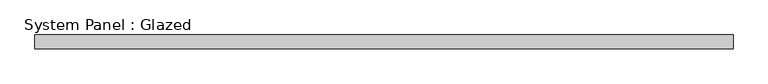
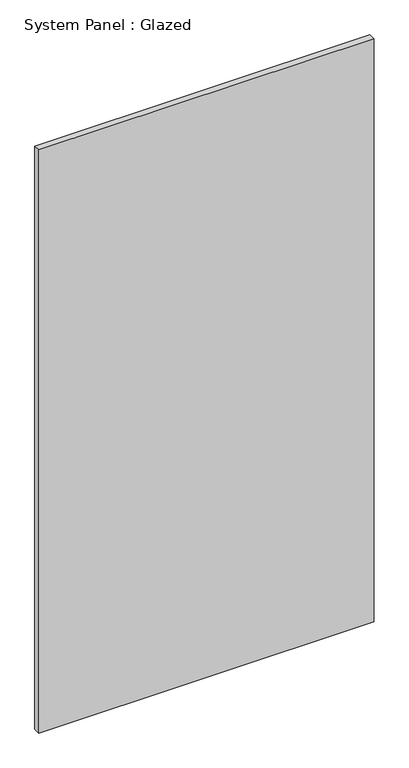
"""IFC4 building model written with IfcOpenShell, lengths in millimetres: plate geometry, System Panel : Glazed."""

from ifc_helpers import new_model, si_unit, origin, origin_with_axes, place, context, project, spatial, polyline, outline, extrude, source, transform, mapped, element, save


def system_panel_glazed_5b896d3e(model_context):
    return source(origin(), model_context, "Body", "SweptSolid", [
        extrude(outline(polyline([(639.2857142, 24.5), (-639.2857142, 24.5), (-639.2857142, 49.5), (639.2857142, 49.5), (639.2857142, 24.5)])), origin_with_axes(), (0.0, 0.0, 1.0), 2350.0),
    ])


if __name__ == "__main__":
    model = new_model("IFC4")
    model_context = context("Model", 3, world=origin())
    ifc_project = project(units=[si_unit("LENGTHUNIT", "METRE", prefix="MILLI")], contexts=[model_context])
    site = spatial("IfcSite", under=ifc_project)
    building = spatial("IfcBuilding", under=site)
    placement = place(None, origin())
    system_panel_glazed_shape = system_panel_glazed_5b896d3e(model_context)
    element("IfcPlate", 1, ObjectType="System Panel : Glazed", at=placement, inside=building, context=model_context, shape_type="MappedRepresentation", body=[
        mapped(system_panel_glazed_shape, transform((0.0, 0.0, 0.0), x_axis=(1.0, 0.0, 0.0), y_axis=(0.0, 1.0, 0.0), z_axis=(0.0, 0.0, 1.0))),
    ])
    save(model, "model.ifc")

# Revit data of these elements
# Type "System Panel : Glazed"
#   Construction Type Id = "GSP4R"
#   Analytic Construction = "1/8 in Pilkington single glazing"
#   Visual Light Transmittance = 0.9
#   Solar Heat Gain Coefficient = 0.86
#   Heat Transfer Coefficient (U) = 6.7069 W/(m²·K)
#   Define Thermal Properties by = 1
# Element 1 (IfcPlate, "System Panel : Glazed")
#   Materials on its faces: "Glass"
# Materials
#   "Glass": class "Glass", colour RGB 0 128 192, transparency 0.75, Description = "Soda Lime Glass", Cost = 0
